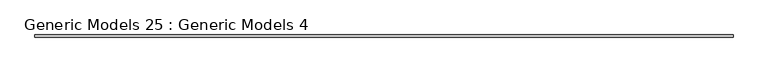
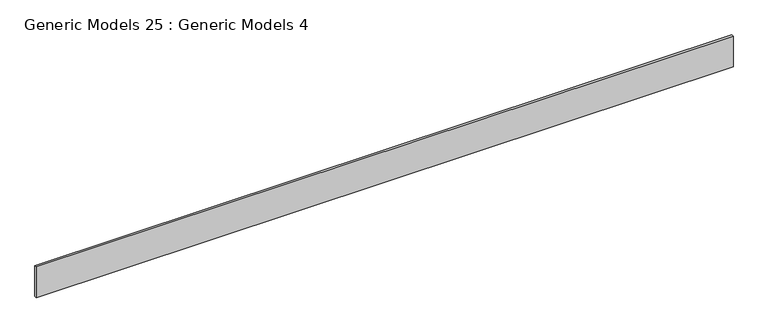
"""IFC4 building model written with IfcOpenShell, lengths in millimetres: proxy geometry, Generic Models 25 : Generic Models 4."""

from ifc_helpers import new_model, si_unit, frame, origin, place, context, project, spatial, polyline, outline, extrude, source, transform, mapped, element, save


def generic_models_25_generic_models_4_194737f7(model_context):
    return source(origin(), model_context, "Body", "SweptSolid", [
        extrude(outline(polyline([(-2310.0733486, -29089.2060818), (-2310.0733486, -29108.2560818), (-8500.0048466, -29108.2560818), (-8500.0048466, -29089.2060818), (-2310.0733486, -29089.2060818)])), frame((0.0, 0.0, 126214.027214), z_axis=(0.0, 0.0, 1.0), x_axis=(1.0, 0.0, 0.0)), (0.0, 0.0, 1.0), 289.0667371),
    ])


if __name__ == "__main__":
    model = new_model("IFC4")
    model_context = context("Model", 3, world=origin())
    ifc_project = project(units=[si_unit("LENGTHUNIT", "METRE", prefix="MILLI")], contexts=[model_context])
    site = spatial("IfcSite", under=ifc_project)
    building = spatial("IfcBuilding", under=site)
    placement = place(None, origin())
    generic_models_25_generic_models_4_shape = generic_models_25_generic_models_4_194737f7(model_context)
    element("IfcBuildingElementProxy", 1, Name="Generic Models 25 : Generic Models 4", ObjectType="Generic Models 25 : Generic Models 4", at=placement, inside=building, context=model_context, shape_type="MappedRepresentation", body=[
        mapped(generic_models_25_generic_models_4_shape, transform((0.0, 0.0, 0.0), x_axis=(1.0, 0.0, 0.0), y_axis=(0.0, 1.0, 0.0), z_axis=(0.0, 0.0, 1.0))),
    ])
    save(model, "model.ifc")

# Revit data of these elements
# Element 1 (IfcBuildingElementProxy, "Generic Models 25 : Generic Models 4")
#   Materials on its faces: "_CDX PLYWOOD - SEE STRUCT DWGs"
# Materials
#   "_CDX PLYWOOD - SEE STRUCT DWGs": class "Generic", colour RGB 98 75 74, transparency 0, Cost = 0
